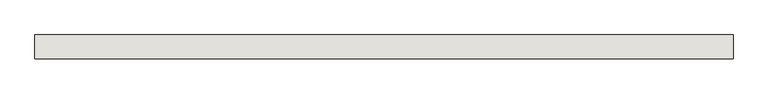
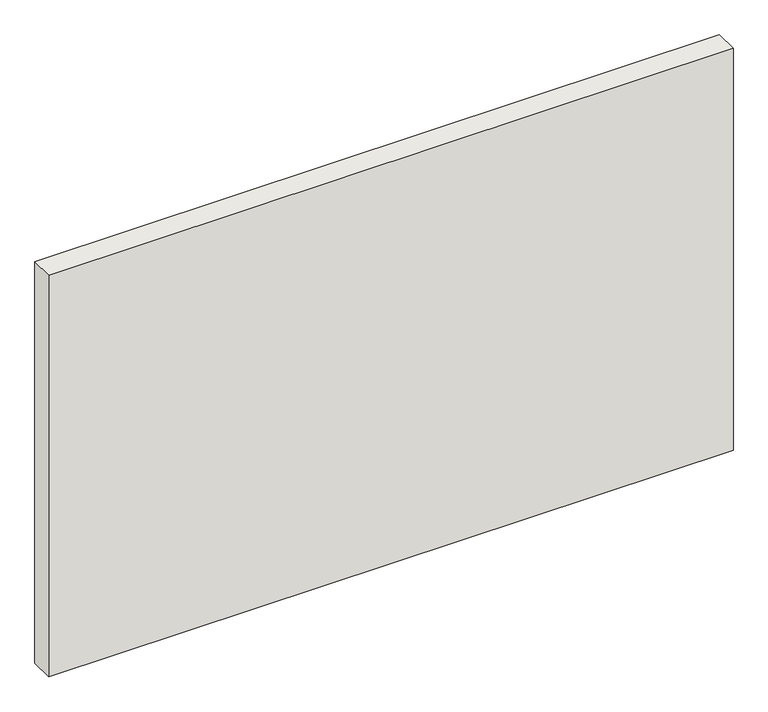
"""IFC4 building model written with IfcOpenShell, lengths in millimetres: wall geometry, Holzwand."""

from ifc_helpers import new_model, si_unit, origin, origin_with_axes, place, context, project, spatial, polyline, outline, extrude, source, transform, mapped, element, save


def wall_c856765b(model_context):
    return source(origin(), model_context, "Body", "SweptSolid", [
        extrude(outline(polyline([(4642.0, 160.0), (4642.0, 0.0), (0.0, 0.0), (0.0, 160.0), (4642.0, 160.0)])), origin_with_axes(), (0.0, 0.0, 1.0), 2880.0),
    ])


if __name__ == "__main__":
    model = new_model("IFC4")
    model_context = context("Model", 3, world=origin())
    ifc_project = project(units=[si_unit("LENGTHUNIT", "METRE", prefix="MILLI")], contexts=[model_context])
    site = spatial("IfcSite", under=ifc_project)
    building = spatial("IfcBuilding", under=site)
    placement = place(None, origin())
    wall_shape = wall_c856765b(model_context)
    element("IfcWall", 1, ObjectType="Holzwand", at=placement, inside=building, context=model_context, shape_type="MappedRepresentation", body=[
        mapped(wall_shape, transform((0.0, 0.0, 0.0), x_axis=(1.0, 0.0, 0.0), y_axis=(0.0, 1.0, 0.0), z_axis=(0.0, 0.0, 1.0))),
    ])
    save(model, "model.ifc")

# Revit data of these elements
# Element 1 (IfcWall, "Holzwand")
#   Materials on its faces: "holzschalung"
# Materials
#   "holzschalung": class "Unassigned", colour RGB 128 128 128, transparency 0
